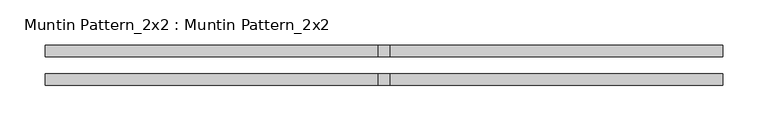
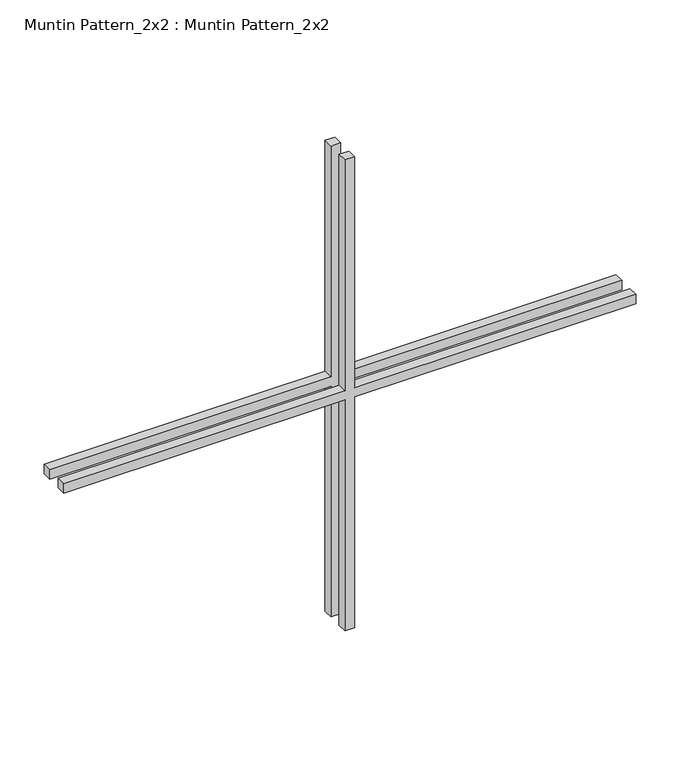
"""IFC4 building model written with IfcOpenShell, lengths in millimetres: proxy geometry, Muntin Pattern_2x2 : Muntin Pattern_2x2."""

import ifcopenshell
import ifcopenshell.guid

model = None  # the IFC model being written
_history = None  # IfcOwnerHistory: only IFC2X3 demands one
_inside = {}  # id of a spatial element -> (the spatial element, [elements in it])
_under = {}  # id of a project, library or spatial element -> (it, [spatial elements below it])
_declared = {}  # id of a project -> (the project, [libraries it declares])
_typed = {}  # id of a type object -> (the type object, [elements of that type])
_made_of = {}  # id of a material, layer set ... -> (it, [elements and type objects made of it])


def new_model(schema):
    """Start an empty IFC model of exactly this schema.

    Asked for "IFC4X3", IfcOpenShell would pick the latest addendum, in which some entities
    have other attributes; the version numbers below select the first issue.
    IFC2X3 requires an IfcOwnerHistory on every rooted entity: one is made here for all.
    """
    global model, _history
    if schema == "IFC4X3":
        model = ifcopenshell.file(schema_version=(4, 3, 0, 0))
    else:
        model = ifcopenshell.file(schema=schema)
    _inside.clear()
    _under.clear()
    _declared.clear()
    _typed.clear()
    _made_of.clear()
    _history = None
    if model.schema == "IFC2X3":
        org = make("IfcOrganization", Name="unknown")
        user = make(
            "IfcPersonAndOrganization",
            ThePerson=make("IfcPerson", FamilyName="unknown"),
            TheOrganization=org,
        )
        app = make(
            "IfcApplication",
            ApplicationDeveloper=org,
            Version="unknown",
            ApplicationFullName="unknown",
            ApplicationIdentifier="unknown",
        )
        _history = make(
            "IfcOwnerHistory",
            OwningUser=user,
            OwningApplication=app,
            ChangeAction="ADDED",
            CreationDate=0,
        )
    return model


def make(cls, **values):
    """One entity of the class cls with the attributes given. An attribute that is None is left unset."""
    return model.create_entity(
        cls, **{name: value for name, value in values.items() if value is not None}
    )


def rooted(cls, **values):
    """An entity with a GlobalId (a new one), such as an element, a storey or a relation."""
    return make(cls, GlobalId=ifcopenshell.guid.new(), OwnerHistory=_history, **values)


def si_unit(unit_type, name, prefix=None):
    """IfcSIUnit, for example si_unit("LENGTHUNIT", "METRE", prefix="MILLI")."""
    return make("IfcSIUnit", UnitType=unit_type, Prefix=prefix, Name=name)


def assignment(units):
    """IfcUnitAssignment: the units of a project."""
    return None if units is None else make("IfcUnitAssignment", Units=units)


def point(xyz):
    """IfcCartesianPoint."""
    return None if xyz is None else make("IfcCartesianPoint", Coordinates=xyz)


def direction(xyz):
    """IfcDirection."""
    return None if xyz is None else make("IfcDirection", DirectionRatios=xyz)


def frame(location, z_axis=None, x_axis=None):
    """IfcAxis2Placement3D, a coordinate frame: its origin and axes. An axis left out is left unset."""
    return make(
        "IfcAxis2Placement3D",
        Location=point(location),
        Axis=direction(z_axis),
        RefDirection=direction(x_axis),
    )


def origin():
    """The frame at (0, 0, 0) with its axes left unset."""
    return frame((0.0, 0.0, 0.0))


def place(relative_to, where):
    """IfcLocalPlacement: puts the frame where relative to a parent placement (None: the world)."""
    return make(
        "IfcLocalPlacement", PlacementRelTo=relative_to, RelativePlacement=where
    )


def context(
    kind, dimensions, precision=None, world=None, true_north=None, identifier=None
):
    """IfcGeometricRepresentationContext, for example the 3D "Model" context."""
    return make(
        "IfcGeometricRepresentationContext",
        ContextIdentifier=identifier,
        ContextType=kind,
        CoordinateSpaceDimension=dimensions,
        Precision=precision,
        WorldCoordinateSystem=world,
        TrueNorth=true_north,
    )


def project(units=None, contexts=None):
    """IfcProject with its units and contexts."""
    return rooted(
        "IfcProject",
        Name="project",
        RepresentationContexts=contexts,
        UnitsInContext=assignment(units),
    )


def spatial(cls, under=None, at=None, **own):
    """A site, building, storey or space (cls), placed at a placement, below another one or the project."""
    s = rooted(cls, ObjectPlacement=at, **own)
    if under is not None:
        _under.setdefault(under.id(), (under, []))[1].append(s)
    return s


def polyline(points):
    """IfcPolyline through the points."""
    return make("IfcPolyline", Points=[point(p) for p in points])


def outline(outer, holes=None, kind="AREA"):
    """IfcArbitraryClosedProfileDef: a profile drawn as a closed curve; with holes, ...WithVoids."""
    if holes is None:
        return make("IfcArbitraryClosedProfileDef", ProfileType=kind, OuterCurve=outer)
    return make(
        "IfcArbitraryProfileDefWithVoids",
        ProfileType=kind,
        OuterCurve=outer,
        InnerCurves=holes,
    )


def extrude(swept, where, along, depth):
    """IfcExtrudedAreaSolid: the profile swept, set in the frame where, extruded along a direction by depth."""
    return make(
        "IfcExtrudedAreaSolid",
        SweptArea=swept,
        Position=where,
        ExtrudedDirection=direction(along),
        Depth=depth,
    )


def shape(context_of_items, identifier, shape_type, items):
    """IfcShapeRepresentation: the items that make up one representation, for example the "Body"."""
    return make(
        "IfcShapeRepresentation",
        ContextOfItems=context_of_items,
        RepresentationIdentifier=identifier,
        RepresentationType=shape_type,
        Items=items,
    )


def source(mapping_origin, context_of_items, identifier, shape_type, items):
    """IfcRepresentationMap: a shape defined once, which mapped items show again and again."""
    return make(
        "IfcRepresentationMap",
        MappingOrigin=mapping_origin,
        MappedRepresentation=shape(context_of_items, identifier, shape_type, items),
    )


def transform(
    local_origin,
    x_axis=None,
    y_axis=None,
    z_axis=None,
    scale=None,
    scale2=None,
    scale3=None,
    uniform=True,
):
    """IfcCartesianTransformationOperator3D, or its non-uniform kind. x_axis, y_axis, z_axis: its Axis1, 2, 3."""
    if uniform:
        return make(
            "IfcCartesianTransformationOperator3D",
            Axis1=direction(x_axis),
            Axis2=direction(y_axis),
            LocalOrigin=point(local_origin),
            Scale=scale,
            Axis3=direction(z_axis),
        )
    return make(
        "IfcCartesianTransformationOperator3DnonUniform",
        Axis1=direction(x_axis),
        Axis2=direction(y_axis),
        LocalOrigin=point(local_origin),
        Scale=scale,
        Axis3=direction(z_axis),
        Scale2=scale2,
        Scale3=scale3,
    )


def mapped(mapping_source, mapping_target):
    """IfcMappedItem: shows the shape of a source again, moved by a transform."""
    return make(
        "IfcMappedItem", MappingSource=mapping_source, MappingTarget=mapping_target
    )


def made_of(thing, what):
    """Note that an element or type object is made of a material, layer set ...; save() writes the relation."""
    if what is not None:
        _made_of.setdefault(what.id(), (what, []))[1].append(thing)
    return thing


def element(
    cls,
    number,
    at=None,
    inside=None,
    cuts=None,
    type_object=None,
    material=None,
    context=None,
    identifier="Body",
    shape_type=None,
    held_by="IfcProductDefinitionShape",
    body=None,
    shapes=None,
    **own,
):
    """One element of the class cls, such as IfcWall. Its Tag is "e" and its number.

    at: its placement. inside: the storey or other place that contains it. cuts: it is an
    opening in that element (IfcRelVoidsElement). A single representation is given by context,
    identifier, shape_type and body (its items); several are given by shapes. held_by: the class
    of the entity that holds the representations. save() writes the other relations.
    """
    e = rooted(cls, Tag="e%d" % number, ObjectPlacement=at, **own)
    if body is not None:
        shapes = [shape(context, identifier, shape_type, body)]
    if shapes is not None:
        e.Representation = make(held_by, Representations=shapes)
    if inside is not None:
        _inside.setdefault(inside.id(), (inside, []))[1].append(e)
    if cuts is not None:
        rooted(
            "IfcRelVoidsElement", RelatingBuildingElement=cuts, RelatedOpeningElement=e
        )
    if type_object is not None:
        _typed.setdefault(type_object.id(), (type_object, []))[1].append(e)
    return made_of(e, material)


def aggregate(whole, parts):
    """IfcRelAggregates: a whole, such as a stair, and the parts it consists of."""
    return rooted("IfcRelAggregates", RelatingObject=whole, RelatedObjects=parts)


def save(model, path):
    """Write the relations noted so far, then the file.

    IfcRelAggregates (storeys below a building ...), IfcRelContainedInSpatialStructure (elements
    in a storey), IfcRelDefinesByType, IfcRelAssociatesMaterial and IfcRelDeclares: one each for
    every whole, place, type object, material and project.
    """
    for whole, parts in _under.values():
        aggregate(whole, parts)
    for where, things in _inside.values():
        rooted(
            "IfcRelContainedInSpatialStructure",
            RelatedElements=things,
            RelatingStructure=where,
        )
    for kind, things in _typed.values():
        rooted("IfcRelDefinesByType", RelatedObjects=things, RelatingType=kind)
    for what, things in _made_of.values():
        rooted("IfcRelAssociatesMaterial", RelatedObjects=things, RelatingMaterial=what)
    for by, libraries in _declared.values():
        rooted("IfcRelDeclares", RelatingContext=by, RelatedDefinitions=libraries)
    model.write(path)


def muntin_pattern_2x2_muntin_pattern_2x2_4af12bc4(model_context):
    return source(origin(), model_context, "Body", "SweptSolid", [
        extrude(outline(polyline([(332.1375, -6.35), (332.1375, -374.59375), (319.4375, -374.59375), (319.4375, -6.35), (0.0, -6.35), (0.0, 6.35), (319.4375, 6.35), (319.4375, 374.59375), (332.1375, 374.59375), (332.1375, 6.35), (651.575, 6.35), (651.575, -6.35), (332.1375, -6.35)])), frame((0.0, -22.225, 0.0), z_axis=(0.0, 1.0, 0.0), x_axis=(0.0, 0.0, 1.0)), (0.0, 0.0, 1.0), 12.7),
        extrude(outline(polyline([(332.1375, -6.35), (332.1375, -374.59375), (319.4375, -374.59375), (319.4375, -6.35), (0.0, -6.35), (0.0, 6.35), (319.4375, 6.35), (319.4375, 374.59375), (332.1375, 374.59375), (332.1375, 6.35), (651.575, 6.35), (651.575, -6.35), (332.1375, -6.35)])), frame((0.0, 9.525, 0.0), z_axis=(0.0, 1.0, 0.0), x_axis=(0.0, 0.0, 1.0)), (0.0, 0.0, 1.0), 12.7),
    ])


if __name__ == "__main__":
    model = new_model("IFC4")
    model_context = context("Model", 3, world=origin())
    ifc_project = project(units=[si_unit("LENGTHUNIT", "METRE", prefix="MILLI")], contexts=[model_context])
    site = spatial("IfcSite", under=ifc_project)
    building = spatial("IfcBuilding", under=site)
    placement = place(None, origin())
    muntin_pattern_2x2_muntin_pattern_2x2_shape = muntin_pattern_2x2_muntin_pattern_2x2_4af12bc4(model_context)
    element("IfcBuildingElementProxy", 1, Name="Muntin Pattern_2x2 : Muntin Pattern_2x2", ObjectType="Muntin Pattern_2x2 : Muntin Pattern_2x2", at=placement, inside=building, context=model_context, shape_type="MappedRepresentation", body=[
        mapped(muntin_pattern_2x2_muntin_pattern_2x2_shape, transform((0.0, 0.0, 0.0), x_axis=(1.0, 0.0, 0.0), y_axis=(0.0, 1.0, 0.0), z_axis=(0.0, 0.0, 1.0))),
    ])
    save(model, "model.ifc")

# Revit data of these elements
# Type "Muntin Pattern_2x2 : Muntin Pattern_2x2"
#   Width [instance default] = 121.92 cm
#   Thickness = 1.27 cm
#   Height [instance default] = 121.92 cm
#   Distance = 1.905 cm
#   Interior Material [instance default] = none
#   Exterior Material [instance default] = none
# Element 1 (IfcBuildingElementProxy, "Muntin Pattern_2x2 : Muntin Pattern_2x2")
#   Width = 74.9188 cm
#   Height = 65.1575 cm
#   Interior Material = Wood - Stained
#   Exterior Material = Clad - White
#   Materials on its faces: "Clad - White", "Wood - Stained"
# Materials
#   "Clad - White": class "Wood", colour RGB 242 242 238, transparency 0, Cost = 0
#   "Wood - Stained": class "Wood", colour RGB 224 178 126, transparency 0, Cost = 0
